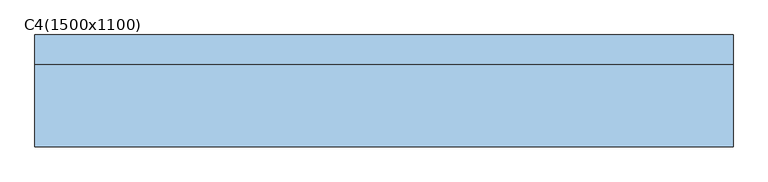
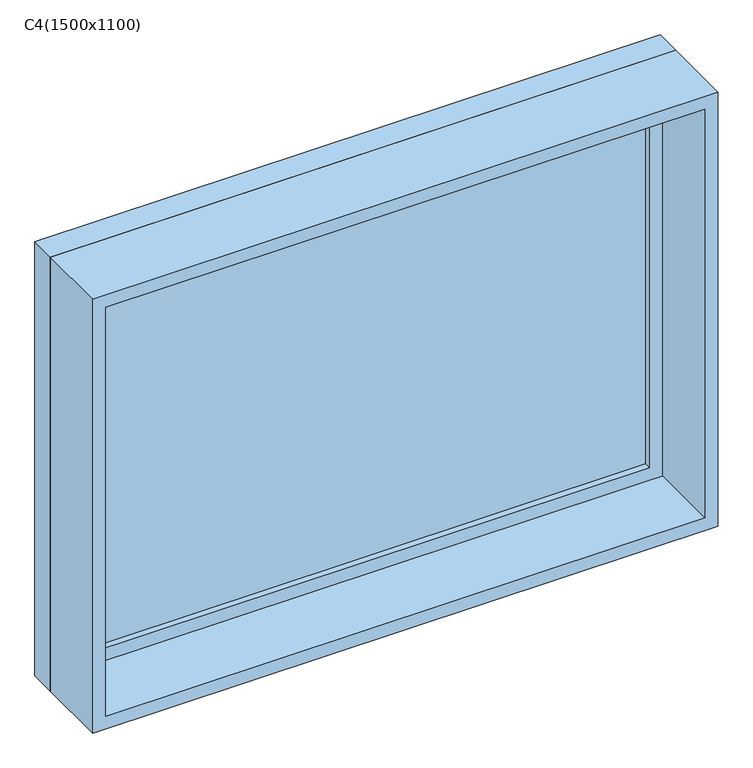
"""IFC4 building model written with IfcOpenShell, lengths in millimetres: window geometry, 固定窗 : C4(1500x1100)."""

from ifc_helpers import new_model, si_unit, frame, origin, place, context, project, spatial, polyline, outline, extrude, source, transform, mapped, element, save


def c4_1500x1100_84ff0e9f(model_context):
    return source(origin(), model_context, "Body", "SweptSolid", [
        extrude(outline(polyline([(648.4, 71.425), (-724.6, 71.425), (-724.6, 84.125), (648.4, 84.125), (648.4, 71.425)])), frame((0.0, 0.0, 963.5), z_axis=(0.0, 0.0, 1.0), x_axis=(1.0, 0.0, 0.0)), (0.0, 0.0, 1.0), 973.0),
        extrude(outline(polyline([(1980.95, -769.05), (919.05, -769.05), (919.05, 692.85), (1980.95, 692.85), (1980.95, -769.05)]), holes=[polyline([(1936.5, -724.6), (1936.5, 648.4), (963.5, 648.4), (963.5, -724.6), (1936.5, -724.6)])]), frame((0.0, 55.55, 0.0), z_axis=(0.0, 1.0, 0.0), x_axis=(0.0, 0.0, 1.0)), (0.0, 0.0, 1.0), 44.45),
        extrude(outline(polyline([(2000.0, -788.1), (900.0, -788.1), (900.0, 711.9), (2000.0, 711.9), (2000.0, -788.1)]), holes=[polyline([(1968.25, -756.35), (1968.25, 680.15), (931.75, 680.15), (931.75, -756.35), (1968.25, -756.35)])]), frame((0.0, -120.0, 0.0), z_axis=(0.0, 1.0, 0.0), x_axis=(0.0, 0.0, 1.0)), (0.0, 0.0, 1.0), 175.55),
        extrude(outline(polyline([(2000.0, 711.9), (2000.0, -788.1), (900.0, -788.1), (900.0, 711.9), (2000.0, 711.9)]), holes=[polyline([(1980.95, 692.85), (919.05, 692.85), (919.05, -769.05), (1980.95, -769.05), (1980.95, 692.85)])]), frame((0.0, 55.55, 0.0), z_axis=(0.0, 1.0, 0.0), x_axis=(0.0, 0.0, 1.0)), (0.0, 0.0, 1.0), 64.45),
    ])


if __name__ == "__main__":
    model = new_model("IFC4")
    model_context = context("Model", 3, world=origin())
    ifc_project = project(units=[si_unit("LENGTHUNIT", "METRE", prefix="MILLI")], contexts=[model_context])
    site = spatial("IfcSite", under=ifc_project)
    building = spatial("IfcBuilding", under=site)
    placement = place(None, origin())
    c4_1500x1100_shape = c4_1500x1100_84ff0e9f(model_context)
    element("IfcWindow", 1, ObjectType="固定窗 : C4(1500x1100)", at=placement, inside=building, context=model_context, shape_type="MappedRepresentation", body=[
        mapped(c4_1500x1100_shape, transform((0.0, 0.0, 0.0), x_axis=(1.0, 0.0, 0.0), y_axis=(0.0, 1.0, 0.0), z_axis=(0.0, 0.0, 1.0))),
    ])
    save(model, "model.ifc")

# Revit data of these elements
# Type "固定窗 : C4(1500x1100)"
#   Type Mark = "C1519"
#   Construction Type Id = "SGL"
#   Analytic Construction = "大型单层玻璃窗"
#   Visual Light Transmittance = 0.9
#   Solar Heat Gain Coefficient = 0.86
#   Rough Width = 1500 mm
#   Rough Height = 1100 mm
#   Heat Transfer Coefficient (U) = 5.5617 W/(m²·K)
#   Height = 1100 mm
#   默认窗台高度 = 900 mm
#   Width = 1500 mm
#   窗嵌入 = 20 mm
#   高窗平面 [instance default] = no
#   通用窗平面 [instance default] = yes
#   玻璃 = none
#   框架材质 = none
#   Wall Closure = (empty or 0)
# Element 1 (IfcWindow, "固定窗 : C4(1500x1100)")
#   Materials on its faces: "玻璃"
# Materials
#   "玻璃": class "玻璃", colour RGB 0 128 192, transparency 0.9, Description = "钠钙玻璃", Cost = 0
